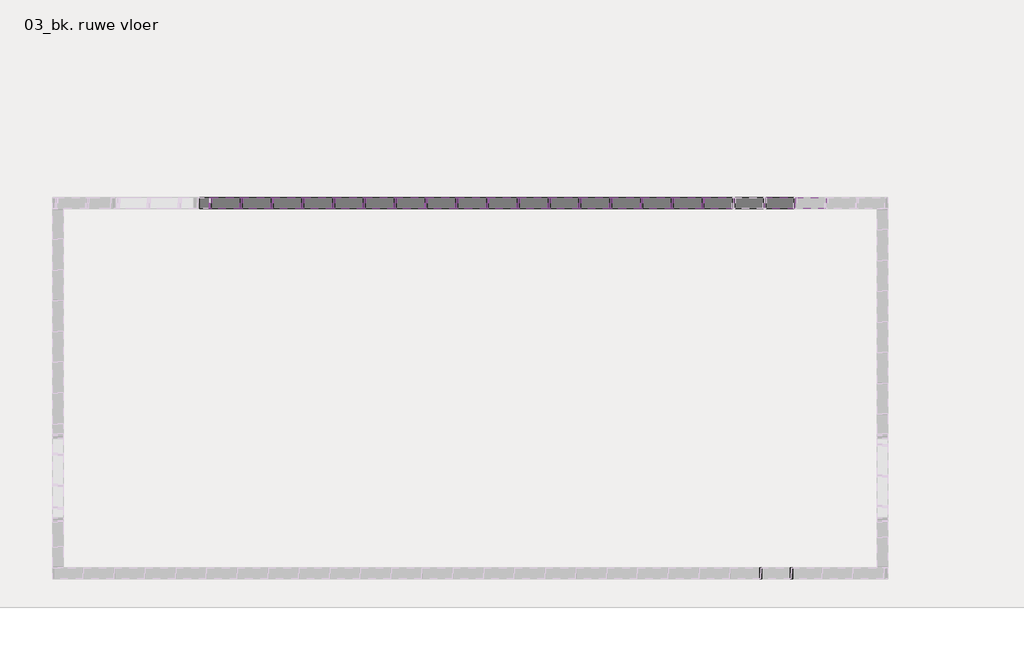
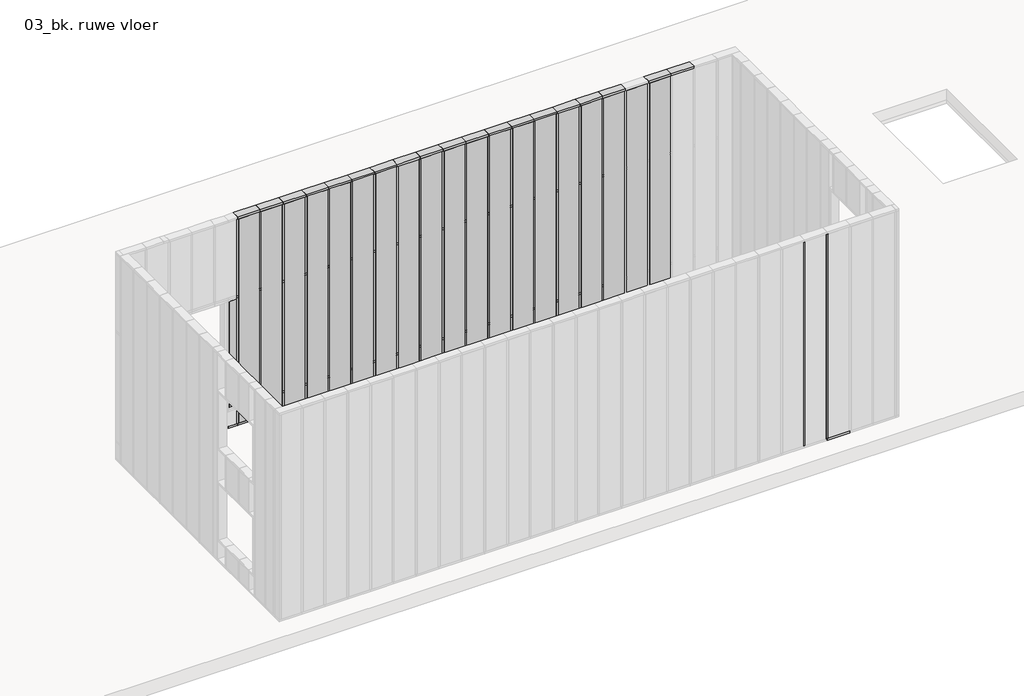
# One storey, part 3 of 9: 124 members, 20 plates.
# Revit data of these elements (continued)
# Type "Rectangular Mullion : NLRS_21_CWM_hsb-regel 38x142_gen_rsf"
#   Export Type to IFC As = "IfcWall"
#   Type IfcGUID = "07M7mRoiH1CR8m_RSKIwpF"
#   Assembly Code = "21.10"
#   built-in parameter 1007322 = 0.465879 (stored number, unit not read)
#   built-in parameter 1007321 = 0.062336 (stored number, unit not read)
#   built-in parameter 1007320 = 0.062336 (stored number, unit not read)
# Type "System Panel : NLRS_21_CWP_hsb-vulling minerale wol 142 _gen_rsf"
#   Export Type to IFC As = "IfcWall"
#   Type IfcGUID = "07M7mRoiH1CR8m_RSKIwpC"
#   Assembly Code = "21.23"
# Element 1 (IfcMember, "Rectangular Mullion : NLRS_21_CWM_hsb-regel 38x142_gen_rsf")
#   IfcGUID = "07M7mRoiH1CR8m_RSKIwQK"
#   IsExternal = yes
#   LoadBearing = yes
#   Phase Created = NLRS_nieuw
#   Materials on its faces: "NLRS_i2_hout naaldhout vuren_gen_rsf"
# Element 2 (IfcMember, "Rectangular Mullion : NLRS_21_CWM_hsb-regel 38x142_gen_rsf")
#   IfcGUID = "07M7mRoiH1CR8m_RSKIwQR"
#   IsExternal = yes
#   LoadBearing = yes
#   Phase Created = NLRS_nieuw
#   Materials on its faces: "NLRS_i2_hout naaldhout vuren_gen_rsf"
# Element 3 (IfcMember, "Rectangular Mullion : NLRS_21_CWM_hsb-regel 38x142_gen_rsf")
#   IfcGUID = "07M7mRoiH1CR8m_RSKIwQP"
#   IsExternal = yes
#   LoadBearing = yes
#   Phase Created = NLRS_nieuw
#   Materials on its faces: "NLRS_i2_hout naaldhout vuren_gen_rsf"
# Element 4 (IfcMember, "Rectangular Mullion : NLRS_21_CWM_hsb-regel 38x142_gen_rsf")
#   IfcGUID = "07M7mRoiH1CR8m_RSKIwQO"
#   IsExternal = yes
#   LoadBearing = yes
#   Phase Created = NLRS_nieuw
#   Materials on its faces: "NLRS_i2_hout naaldhout vuren_gen_rsf"
# Element 5 (IfcMember, "Rectangular Mullion : NLRS_21_CWM_hsb-regel 38x142_gen_rsf")
#   IfcGUID = "07M7mRoiH1CR8m_RSKIwQV"
#   IsExternal = yes
#   LoadBearing = yes
#   Phase Created = NLRS_nieuw
#   Materials on its faces: "NLRS_i2_hout naaldhout vuren_gen_rsf"
# Element 6 (IfcMember, "Rectangular Mullion : NLRS_21_CWM_hsb-regel 38x142_gen_rsf")
#   IfcGUID = "07M7mRoiH1CR8m_RSKIwQU"
#   IsExternal = yes
#   LoadBearing = yes
#   Phase Created = NLRS_nieuw
#   Materials on its faces: "NLRS_i2_hout naaldhout vuren_gen_rsf"
# Element 7 (IfcMember, "Rectangular Mullion : NLRS_21_CWM_hsb-regel 38x142_gen_rsf")
#   IfcGUID = "07M7mRoiH1CR8m_RSKIwQT"
#   IsExternal = yes
#   LoadBearing = yes
#   Phase Created = NLRS_nieuw
#   Materials on its faces: "NLRS_i2_hout naaldhout vuren_gen_rsf"
# Element 8 (IfcMember, "Rectangular Mullion : NLRS_21_CWM_hsb-regel 38x142_gen_rsf")
#   IfcGUID = "07M7mRoiH1CR8m_RSKIwQS"
#   IsExternal = yes
#   LoadBearing = yes
#   Phase Created = NLRS_nieuw
#   Materials on its faces: "NLRS_i2_hout naaldhout vuren_gen_rsf"
# Element 9 (IfcMember, "Rectangular Mullion : NLRS_21_CWM_hsb-regel 38x142_gen_rsf")
#   IfcGUID = "07M7mRoiH1CR8m_RSKIwPZ"
#   IsExternal = yes
#   LoadBearing = yes
#   Phase Created = NLRS_nieuw
#   Materials on its faces: "NLRS_i2_hout naaldhout vuren_gen_rsf"
# Element 10 (IfcMember, "Rectangular Mullion : NLRS_21_CWM_hsb-regel 38x142_gen_rsf")
#   IfcGUID = "07M7mRoiH1CR8m_RSKIwPY"
#   IsExternal = yes
#   LoadBearing = yes
#   Phase Created = NLRS_nieuw
#   Materials on its faces: "NLRS_i2_hout naaldhout vuren_gen_rsf"
# Element 11 (IfcMember, "Rectangular Mullion : NLRS_21_CWM_hsb-regel 38x142_gen_rsf")
#   IfcGUID = "07M7mRoiH1CR8m_RSKIwPX"
#   IsExternal = yes
#   LoadBearing = yes
#   Phase Created = NLRS_nieuw
#   Materials on its faces: "NLRS_i2_hout naaldhout vuren_gen_rsf"
# Element 12 (IfcMember, "Rectangular Mullion : NLRS_21_CWM_hsb-regel 38x142_gen_rsf")
#   IfcGUID = "07M7mRoiH1CR8m_RSKIwPW"
#   IsExternal = yes
#   LoadBearing = yes
#   Phase Created = NLRS_nieuw
#   Materials on its faces: "NLRS_i2_hout naaldhout vuren_gen_rsf"
# Element 13 (IfcMember, "Rectangular Mullion : NLRS_21_CWM_hsb-regel 38x142_gen_rsf")
#   IfcGUID = "07M7mRoiH1CR8m_RSKIwPd"
#   IsExternal = yes
#   LoadBearing = yes
#   Phase Created = NLRS_nieuw
#   Materials on its faces: "NLRS_i2_hout naaldhout vuren_gen_rsf"
# Element 14 (IfcMember, "Rectangular Mullion : NLRS_21_CWM_hsb-regel 38x142_gen_rsf")
#   IfcGUID = "07M7mRoiH1CR8m_RSKIwPc"
#   IsExternal = yes
#   LoadBearing = yes
#   Phase Created = NLRS_nieuw
#   Materials on its faces: "NLRS_i2_hout naaldhout vuren_gen_rsf"
# Element 15 (IfcMember, "Rectangular Mullion : NLRS_21_CWM_hsb-regel 38x142_gen_rsf")
#   IfcGUID = "07M7mRoiH1CR8m_RSKIwPb"
#   IsExternal = yes
#   LoadBearing = yes
#   Phase Created = NLRS_nieuw
#   Materials on its faces: "NLRS_i2_hout naaldhout vuren_gen_rsf"
# Element 16 (IfcMember, "Rectangular Mullion : NLRS_21_CWM_hsb-regel 38x142_gen_rsf")
#   IfcGUID = "07M7mRoiH1CR8m_RSKIwPa"
#   IsExternal = yes
#   LoadBearing = yes
#   Phase Created = NLRS_nieuw
#   Materials on its faces: "NLRS_i2_hout naaldhout vuren_gen_rsf"
# Element 17 (IfcMember, "Rectangular Mullion : NLRS_21_CWM_hsb-regel 38x142_gen_rsf")
#   IfcGUID = "07M7mRoiH1CR8m_RSKIwUD"
#   IsExternal = yes
#   LoadBearing = yes
#   Phase Created = NLRS_nieuw
#   Materials on its faces: "NLRS_i2_hout naaldhout vuren_gen_rsf"
# Element 18 (IfcMember, "Rectangular Mullion : NLRS_21_CWM_hsb-regel 38x142_gen_rsf")
#   IfcGUID = "07M7mRoiH1CR8m_RSKIwUC"
#   IsExternal = yes
#   LoadBearing = yes
#   Phase Created = NLRS_nieuw
#   Materials on its faces: "NLRS_i2_hout naaldhout vuren_gen_rsf"
# Element 19 (IfcMember, "Rectangular Mullion : NLRS_21_CWM_hsb-regel 38x142_gen_rsf")
#   IfcGUID = "07M7mRoiH1CR8m_RSKIwIM"
#   IsExternal = yes
#   LoadBearing = yes
#   Phase Created = NLRS_nieuw
#   Materials on its faces: "NLRS_i2_hout naaldhout vuren_gen_rsf"
# Element 20 (IfcMember, "Rectangular Mullion : NLRS_21_CWM_hsb-regel 38x142_gen_rsf")
#   IfcGUID = "07M7mRoiH1CR8m_RSKIwPj"
#   IsExternal = yes
#   LoadBearing = yes
#   Phase Created = NLRS_nieuw
#   Materials on its faces: "NLRS_i2_hout naaldhout vuren_gen_rsf"
# Element 21 (IfcMember, "Rectangular Mullion : NLRS_21_CWM_hsb-regel 38x142_gen_rsf")
#   IfcGUID = "07M7mRoiH1CR8m_RSKIwPi"
#   IsExternal = yes
#   LoadBearing = yes
#   Phase Created = NLRS_nieuw
#   Materials on its faces: "NLRS_i2_hout naaldhout vuren_gen_rsf"
# Element 22 (IfcMember, "Rectangular Mullion : NLRS_21_CWM_hsb-regel 38x142_gen_rsf")
#   IfcGUID = "07M7mRoiH1CR8m_RSKIwPp"
#   IsExternal = yes
#   LoadBearing = yes
#   Phase Created = NLRS_nieuw
#   Materials on its faces: "NLRS_i2_hout naaldhout vuren_gen_rsf"
# Element 23 (IfcMember, "Rectangular Mullion : NLRS_21_CWM_hsb-regel 38x142_gen_rsf")
#   IfcGUID = "07M7mRoiH1CR8m_RSKIwPo"
#   IsExternal = yes
#   LoadBearing = yes
#   Phase Created = NLRS_nieuw
#   Materials on its faces: "NLRS_i2_hout naaldhout vuren_gen_rsf"
# Element 24 (IfcMember, "Rectangular Mullion : NLRS_21_CWM_hsb-regel 38x142_gen_rsf")
#   IfcGUID = "07M7mRoiH1CR8m_RSKIwPn"
#   IsExternal = yes
#   LoadBearing = yes
#   Phase Created = NLRS_nieuw
#   Materials on its faces: "NLRS_i2_hout naaldhout vuren_gen_rsf"
# Element 25 (IfcMember, "Rectangular Mullion : NLRS_21_CWM_hsb-regel 38x142_gen_rsf")
#   IfcGUID = "07M7mRoiH1CR8m_RSKIwPm"
#   IsExternal = yes
#   LoadBearing = yes
#   Phase Created = NLRS_nieuw
#   Materials on its faces: "NLRS_i2_hout naaldhout vuren_gen_rsf"
# Element 26 (IfcMember, "Rectangular Mullion : NLRS_21_CWM_hsb-regel 38x142_gen_rsf")
#   IfcGUID = "07M7mRoiH1CR8m_RSKIwPt"
#   IsExternal = yes
#   LoadBearing = yes
#   Phase Created = NLRS_nieuw
#   Materials on its faces: "NLRS_i2_hout naaldhout vuren_gen_rsf"
# Element 27 (IfcMember, "Rectangular Mullion : NLRS_21_CWM_hsb-regel 38x142_gen_rsf")
#   IfcGUID = "07M7mRoiH1CR8m_RSKIwPs"
#   IsExternal = yes
#   LoadBearing = yes
#   Phase Created = NLRS_nieuw
#   Materials on its faces: "NLRS_i2_hout naaldhout vuren_gen_rsf"
# Element 28 (IfcMember, "Rectangular Mullion : NLRS_21_CWM_hsb-regel 38x142_gen_rsf")
#   IfcGUID = "07M7mRoiH1CR8m_RSKIwPr"
#   IsExternal = yes
#   LoadBearing = yes
#   Phase Created = NLRS_nieuw
#   Materials on its faces: "NLRS_i2_hout naaldhout vuren_gen_rsf"
# Element 29 (IfcMember, "Rectangular Mullion : NLRS_21_CWM_hsb-regel 38x142_gen_rsf")
#   IfcGUID = "07M7mRoiH1CR8m_RSKIwPq"
#   IsExternal = yes
#   LoadBearing = yes
#   Phase Created = NLRS_nieuw
#   Materials on its faces: "NLRS_i2_hout naaldhout vuren_gen_rsf"
# Element 30 (IfcMember, "Rectangular Mullion : NLRS_21_CWM_hsb-regel 38x142_gen_rsf")
#   IfcGUID = "07M7mRoiH1CR8m_RSKIwPx"
#   IsExternal = yes
#   LoadBearing = yes
#   Phase Created = NLRS_nieuw
#   Materials on its faces: "NLRS_i2_hout naaldhout vuren_gen_rsf"
# Element 31 (IfcMember, "Rectangular Mullion : NLRS_21_CWM_hsb-regel 38x142_gen_rsf")
#   IfcGUID = "07M7mRoiH1CR8m_RSKIwPw"
#   IsExternal = yes
#   LoadBearing = yes
#   Phase Created = NLRS_nieuw
#   Materials on its faces: "NLRS_i2_hout naaldhout vuren_gen_rsf"
# Element 32 (IfcMember, "Rectangular Mullion : NLRS_21_CWM_hsb-regel 38x142_gen_rsf")
#   IfcGUID = "07M7mRoiH1CR8m_RSKIwPv"
#   IsExternal = yes
#   LoadBearing = yes
#   Phase Created = NLRS_nieuw
#   Materials on its faces: "NLRS_i2_hout naaldhout vuren_gen_rsf"
# Element 33 (IfcMember, "Rectangular Mullion : NLRS_21_CWM_hsb-regel 38x142_gen_rsf")
#   IfcGUID = "07M7mRoiH1CR8m_RSKIwPu"
#   IsExternal = yes
#   LoadBearing = yes
#   Phase Created = NLRS_nieuw
#   Materials on its faces: "NLRS_i2_hout naaldhout vuren_gen_rsf"
# Element 34 (IfcMember, "Rectangular Mullion : NLRS_21_CWM_hsb-regel 38x142_gen_rsf")
#   IfcGUID = "07M7mRoiH1CR8m_RSKIwUJ"
#   IsExternal = yes
#   LoadBearing = yes
#   Phase Created = NLRS_nieuw
#   Materials on its faces: "NLRS_i2_hout naaldhout vuren_gen_rsf"
# Element 35 (IfcMember, "Rectangular Mullion : NLRS_21_CWM_hsb-regel 38x142_gen_rsf")
#   IfcGUID = "07M7mRoiH1CR8m_RSKIwJV"
#   IsExternal = yes
#   LoadBearing = yes
#   Phase Created = NLRS_nieuw
#   Materials on its faces: "NLRS_i2_hout naaldhout vuren_gen_rsf"
# Element 36 (IfcMember, "Rectangular Mullion : NLRS_21_CWM_hsb-regel 38x142_gen_rsf")
#   IfcGUID = "3JRv6RmLn4$9gi2tFo70EI"
#   IsExternal = yes
#   LoadBearing = yes
#   Phase Created = NLRS_nieuw
#   Materials on its faces: "NLRS_i2_hout naaldhout vuren_gen_rsf"
# Element 37 (IfcMember, "Rectangular Mullion : NLRS_21_CWM_hsb-regel 38x142_gen_rsf")
#   IfcGUID = "07M7mRoiH1CR8m_RSKIwIY"
#   IsExternal = yes
#   LoadBearing = yes
#   Phase Created = NLRS_nieuw
#   Materials on its faces: "NLRS_i2_hout naaldhout vuren_gen_rsf"
# Element 38 (IfcMember, "Rectangular Mullion : NLRS_21_CWM_hsb-regel 38x142_gen_rsf")
#   IfcGUID = "07M7mRoiH1CR8m_RSKIwIX"
#   IsExternal = yes
#   LoadBearing = yes
#   Phase Created = NLRS_nieuw
#   Materials on its faces: "NLRS_i2_hout naaldhout vuren_gen_rsf"
# Element 39 (IfcMember, "Rectangular Mullion : NLRS_21_CWM_hsb-regel 38x142_gen_rsf")
#   IfcGUID = "07M7mRoiH1CR8m_RSKIwP0"
#   IsExternal = yes
#   LoadBearing = yes
#   Phase Created = NLRS_nieuw
#   Materials on its faces: "NLRS_i2_hout naaldhout vuren_gen_rsf"
# Element 40 (IfcMember, "Rectangular Mullion : NLRS_21_CWM_hsb-regel 38x142_gen_rsf")
#   IfcGUID = "07M7mRoiH1CR8m_RSKIwP7"
#   IsExternal = yes
#   LoadBearing = yes
#   Phase Created = NLRS_nieuw
#   Materials on its faces: "NLRS_i2_hout naaldhout vuren_gen_rsf"
# Element 41 (IfcMember, "Rectangular Mullion : NLRS_21_CWM_hsb-regel 38x142_gen_rsf")
#   IfcGUID = "07M7mRoiH1CR8m_RSKIwP6"
#   IsExternal = yes
#   LoadBearing = yes
#   Phase Created = NLRS_nieuw
#   Materials on its faces: "NLRS_i2_hout naaldhout vuren_gen_rsf"
# Element 42 (IfcMember, "Rectangular Mullion : NLRS_21_CWM_hsb-regel 38x142_gen_rsf")
#   IfcGUID = "07M7mRoiH1CR8m_RSKIwP5"
#   IsExternal = yes
#   LoadBearing = yes
#   Phase Created = NLRS_nieuw
#   Materials on its faces: "NLRS_i2_hout naaldhout vuren_gen_rsf"
# Element 43 (IfcMember, "Rectangular Mullion : NLRS_21_CWM_hsb-regel 38x142_gen_rsf")
#   IfcGUID = "07M7mRoiH1CR8m_RSKIwP4"
#   IsExternal = yes
#   LoadBearing = yes
#   Phase Created = NLRS_nieuw
#   Materials on its faces: "NLRS_i2_hout naaldhout vuren_gen_rsf"
# Element 44 (IfcMember, "Rectangular Mullion : NLRS_21_CWM_hsb-regel 38x142_gen_rsf")
#   IfcGUID = "07M7mRoiH1CR8m_RSKIwPB"
#   IsExternal = yes
#   LoadBearing = yes
#   Phase Created = NLRS_nieuw
#   Materials on its faces: "NLRS_i2_hout naaldhout vuren_gen_rsf"
# Element 45 (IfcMember, "Rectangular Mullion : NLRS_21_CWM_hsb-regel 38x142_gen_rsf")
#   IfcGUID = "07M7mRoiH1CR8m_RSKIwPA"
#   IsExternal = yes
#   LoadBearing = yes
#   Phase Created = NLRS_nieuw
#   Materials on its faces: "NLRS_i2_hout naaldhout vuren_gen_rsf"
# Element 46 (IfcMember, "Rectangular Mullion : NLRS_21_CWM_hsb-regel 38x142_gen_rsf")
#   IfcGUID = "07M7mRoiH1CR8m_RSKIwP9"
#   IsExternal = yes
#   LoadBearing = yes
#   Phase Created = NLRS_nieuw
#   Materials on its faces: "NLRS_i2_hout naaldhout vuren_gen_rsf"
# Element 47 (IfcMember, "Rectangular Mullion : NLRS_21_CWM_hsb-regel 38x142_gen_rsf")
#   IfcGUID = "07M7mRoiH1CR8m_RSKIwP8"
#   IsExternal = yes
#   LoadBearing = yes
#   Phase Created = NLRS_nieuw
#   Materials on its faces: "NLRS_i2_hout naaldhout vuren_gen_rsf"
# Element 48 (IfcMember, "Rectangular Mullion : NLRS_21_CWM_hsb-regel 38x142_gen_rsf")
#   IfcGUID = "07M7mRoiH1CR8m_RSKIwPF"
#   IsExternal = yes
#   LoadBearing = yes
#   Phase Created = NLRS_nieuw
#   Materials on its faces: "NLRS_i2_hout naaldhout vuren_gen_rsf"
# Element 49 (IfcMember, "Rectangular Mullion : NLRS_21_CWM_hsb-regel 38x142_gen_rsf")
#   IfcGUID = "07M7mRoiH1CR8m_RSKIwPE"
#   IsExternal = yes
#   LoadBearing = yes
#   Phase Created = NLRS_nieuw
#   Materials on its faces: "NLRS_i2_hout naaldhout vuren_gen_rsf"
# Element 50 (IfcMember, "Rectangular Mullion : NLRS_21_CWM_hsb-regel 38x142_gen_rsf")
#   IfcGUID = "07M7mRoiH1CR8m_RSKIwPD"
#   IsExternal = yes
#   LoadBearing = yes
#   Phase Created = NLRS_nieuw
#   Materials on its faces: "NLRS_i2_hout naaldhout vuren_gen_rsf"
# Element 51 (IfcMember, "Rectangular Mullion : NLRS_21_CWM_hsb-regel 38x142_gen_rsf")
#   IfcGUID = "07M7mRoiH1CR8m_RSKIwPC"
#   IsExternal = yes
#   LoadBearing = yes
#   Phase Created = NLRS_nieuw
#   Materials on its faces: "NLRS_i2_hout naaldhout vuren_gen_rsf"
# Element 52 (IfcMember, "Rectangular Mullion : NLRS_21_CWM_hsb-regel 38x142_gen_rsf")
#   IfcGUID = "07M7mRoiH1CR8m_RSKIwPJ"
#   IsExternal = yes
#   LoadBearing = yes
#   Phase Created = NLRS_nieuw
#   Materials on its faces: "NLRS_i2_hout naaldhout vuren_gen_rsf"
# Element 53 (IfcMember, "Rectangular Mullion : NLRS_21_CWM_hsb-regel 38x142_gen_rsf")
#   IfcGUID = "07M7mRoiH1CR8m_RSKIwUI"
#   IsExternal = yes
#   LoadBearing = yes
#   Phase Created = NLRS_nieuw
#   Materials on its faces: "NLRS_i2_hout naaldhout vuren_gen_rsf"
# Element 54 (IfcMember, "Rectangular Mullion : NLRS_21_CWM_hsb-regel 38x142_gen_rsf")
#   IfcGUID = "07M7mRoiH1CR8m_RSKIwUH"
#   IsExternal = yes
#   LoadBearing = yes
#   Phase Created = NLRS_nieuw
#   Materials on its faces: "NLRS_i2_hout naaldhout vuren_gen_rsf"
# Element 55 (IfcMember, "Rectangular Mullion : NLRS_21_CWM_hsb-regel 38x142_gen_rsf")
#   IfcGUID = "07M7mRoiH1CR8m_RSKIwHY"
#   IsExternal = yes
#   LoadBearing = yes
#   Phase Created = NLRS_nieuw
#   Materials on its faces: "NLRS_i2_hout naaldhout vuren_gen_rsf"
# Element 56 (IfcMember, "Rectangular Mullion : NLRS_21_CWM_hsb-regel 38x142_gen_rsf")
#   IfcGUID = "3JRv6RmLn4$9gi2tFo70EJ"
#   IsExternal = yes
#   LoadBearing = yes
#   Phase Created = NLRS_nieuw
#   Materials on its faces: "NLRS_i2_hout naaldhout vuren_gen_rsf"
# Element 57 (IfcMember, "Rectangular Mullion : NLRS_21_CWM_hsb-regel 38x142_gen_rsf")
#   IfcGUID = "3JRv6RmLn4$9gi2tFo70WL"
#   IsExternal = yes
#   LoadBearing = yes
#   Phase Created = NLRS_nieuw
#   Materials on its faces: "NLRS_i2_hout naaldhout vuren_gen_rsf"
# Element 58 (IfcMember, "Rectangular Mullion : NLRS_21_CWM_hsb-regel 38x142_gen_rsf")
#   IfcGUID = "3JRv6RmLn4$9gi2tFo70WM"
#   IsExternal = yes
#   LoadBearing = yes
#   Phase Created = NLRS_nieuw
#   Materials on its faces: "NLRS_i2_hout naaldhout vuren_gen_rsf"
# Element 59 (IfcMember, "Rectangular Mullion : NLRS_21_CWM_hsb-regel 38x142_gen_rsf")
#   IfcGUID = "3JRv6RmLn4$9gi2tFo70WN"
#   IsExternal = yes
#   LoadBearing = yes
#   Phase Created = NLRS_nieuw
#   Materials on its faces: "NLRS_i2_hout naaldhout vuren_gen_rsf"
# Element 60 (IfcMember, "Rectangular Mullion : NLRS_21_CWM_hsb-regel 38x142_gen_rsf")
#   IfcGUID = "3JRv6RmLn4$9gi2tFo70WG"
#   IsExternal = yes
#   LoadBearing = yes
#   Phase Created = NLRS_nieuw
#   Materials on its faces: "NLRS_i2_hout naaldhout vuren_gen_rsf"
# Element 61 (IfcMember, "Rectangular Mullion : NLRS_21_CWM_hsb-regel 38x142_gen_rsf")
#   IfcGUID = "3JRv6RmLn4$9gi2tFo70WH"
#   IsExternal = yes
#   LoadBearing = yes
#   Phase Created = NLRS_nieuw
#   Materials on its faces: "NLRS_i2_hout naaldhout vuren_gen_rsf"
# Element 62 (IfcMember, "Rectangular Mullion : NLRS_21_CWM_hsb-regel 38x142_gen_rsf")
#   IfcGUID = "3JRv6RmLn4$9gi2tFo70WI"
#   IsExternal = yes
#   LoadBearing = yes
#   Phase Created = NLRS_nieuw
#   Materials on its faces: "NLRS_i2_hout naaldhout vuren_gen_rsf"
# Element 63 (IfcMember, "Rectangular Mullion : NLRS_21_CWM_hsb-regel 38x142_gen_rsf")
#   IfcGUID = "3JRv6RmLn4$9gi2tFo70WJ"
#   IsExternal = yes
#   LoadBearing = yes
#   Phase Created = NLRS_nieuw
#   Materials on its faces: "NLRS_i2_hout naaldhout vuren_gen_rsf"
# Element 64 (IfcMember, "Rectangular Mullion : NLRS_21_CWM_hsb-regel 38x142_gen_rsf")
#   IfcGUID = "3JRv6RmLn4$9gi2tFo70WS"
#   IsExternal = yes
#   LoadBearing = yes
#   Phase Created = NLRS_nieuw
#   Materials on its faces: "NLRS_i2_hout naaldhout vuren_gen_rsf"
# Element 65 (IfcMember, "Rectangular Mullion : NLRS_21_CWM_hsb-regel 38x142_gen_rsf")
#   IfcGUID = "3JRv6RmLn4$9gi2tFo70WT"
#   IsExternal = yes
#   LoadBearing = yes
#   Phase Created = NLRS_nieuw
#   Materials on its faces: "NLRS_i2_hout naaldhout vuren_gen_rsf"
# Element 66 (IfcMember, "Rectangular Mullion : NLRS_21_CWM_hsb-regel 38x142_gen_rsf")
#   IfcGUID = "3JRv6RmLn4$9gi2tFo70WU"
#   IsExternal = yes
#   LoadBearing = yes
#   Phase Created = NLRS_nieuw
#   Materials on its faces: "NLRS_i2_hout naaldhout vuren_gen_rsf"
# Element 67 (IfcMember, "Rectangular Mullion : NLRS_21_CWM_hsb-regel 38x142_gen_rsf")
#   IfcGUID = "3JRv6RmLn4$9gi2tFo70WV"
#   IsExternal = yes
#   LoadBearing = yes
#   Phase Created = NLRS_nieuw
#   Materials on its faces: "NLRS_i2_hout naaldhout vuren_gen_rsf"
# Element 68 (IfcMember, "Rectangular Mullion : NLRS_21_CWM_hsb-regel 38x142_gen_rsf")
#   IfcGUID = "3JRv6RmLn4$9gi2tFo70WO"
#   IsExternal = yes
#   LoadBearing = yes
#   Phase Created = NLRS_nieuw
#   Materials on its faces: "NLRS_i2_hout naaldhout vuren_gen_rsf"
# Element 69 (IfcMember, "Rectangular Mullion : NLRS_21_CWM_hsb-regel 38x142_gen_rsf")
#   IfcGUID = "3JRv6RmLn4$9gi2tFo70WP"
#   IsExternal = yes
#   LoadBearing = yes
#   Phase Created = NLRS_nieuw
#   Materials on its faces: "NLRS_i2_hout naaldhout vuren_gen_rsf"
# Element 70 (IfcMember, "Rectangular Mullion : NLRS_21_CWM_hsb-regel 38x142_gen_rsf")
#   IfcGUID = "3JRv6RmLn4$9gi2tFo70WQ"
#   IsExternal = yes
#   LoadBearing = yes
#   Phase Created = NLRS_nieuw
#   Materials on its faces: "NLRS_i2_hout naaldhout vuren_gen_rsf"
# Element 71 (IfcMember, "Rectangular Mullion : NLRS_21_CWM_hsb-regel 38x142_gen_rsf")
#   IfcGUID = "3JRv6RmLn4$9gi2tFo70WR"
#   IsExternal = yes
#   LoadBearing = yes
#   Phase Created = NLRS_nieuw
#   Materials on its faces: "NLRS_i2_hout naaldhout vuren_gen_rsf"
# Element 72 (IfcMember, "Rectangular Mullion : NLRS_21_CWM_hsb-regel 38x142_gen_rsf")
#   IfcGUID = "3JRv6RmLn4$9gi2tFo70Xa"
#   IsExternal = yes
#   LoadBearing = yes
#   Phase Created = NLRS_nieuw
#   Materials on its faces: "NLRS_i2_hout naaldhout vuren_gen_rsf"
# Element 73 (IfcMember, "Rectangular Mullion : NLRS_21_CWM_hsb-regel 38x142_gen_rsf")
#   IfcGUID = "3JRv6RmLn4$9gi2tFo70Xb"
#   IsExternal = yes
#   LoadBearing = yes
#   Phase Created = NLRS_nieuw
#   Materials on its faces: "NLRS_i2_hout naaldhout vuren_gen_rsf"
# Element 74 (IfcMember, "Rectangular Mullion : NLRS_21_CWM_hsb-regel 38x142_gen_rsf")
#   IfcGUID = "3JRv6RmLn4$9gi2tFo70wj"
#   IsExternal = yes
#   LoadBearing = yes
#   Phase Created = NLRS_nieuw
#   Materials on its faces: "NLRS_i2_hout naaldhout vuren_gen_rsf"
# Element 75 (IfcMember, "Rectangular Mullion : NLRS_21_CWM_hsb-regel 38x142_gen_rsf")
#   IfcGUID = "3JRv6RmLn4$9gi2tFo70wk"
#   IsExternal = yes
#   LoadBearing = yes
#   Phase Created = NLRS_nieuw
#   Materials on its faces: "NLRS_i2_hout naaldhout vuren_gen_rsf"
# Element 76 (IfcMember, "Rectangular Mullion : NLRS_21_CWM_hsb-regel 38x142_gen_rsf")
#   IfcGUID = "3JRv6RmLn4$9gi2tFo70wl"
#   IsExternal = yes
#   LoadBearing = yes
#   Phase Created = NLRS_nieuw
#   Materials on its faces: "NLRS_i2_hout naaldhout vuren_gen_rsf"
# Element 77 (IfcMember, "Rectangular Mullion : NLRS_21_CWM_hsb-regel 38x142_gen_rsf")
#   IfcGUID = "3JRv6RmLn4$9gi2tFo70we"
#   IsExternal = yes
#   LoadBearing = yes
#   Phase Created = NLRS_nieuw
#   Materials on its faces: "NLRS_i2_hout naaldhout vuren_gen_rsf"
# Element 78 (IfcMember, "Rectangular Mullion : NLRS_21_CWM_hsb-regel 38x142_gen_rsf")
#   IfcGUID = "3JRv6RmLn4$9gi2tFo70wf"
#   IsExternal = yes
#   LoadBearing = yes
#   Phase Created = NLRS_nieuw
#   Materials on its faces: "NLRS_i2_hout naaldhout vuren_gen_rsf"
# Element 79 (IfcMember, "Rectangular Mullion : NLRS_21_CWM_hsb-regel 38x142_gen_rsf")
#   IfcGUID = "3JRv6RmLn4$9gi2tFo70wg"
#   IsExternal = yes
#   LoadBearing = yes
#   Phase Created = NLRS_nieuw
#   Materials on its faces: "NLRS_i2_hout naaldhout vuren_gen_rsf"
# Element 80 (IfcMember, "Rectangular Mullion : NLRS_21_CWM_hsb-regel 38x142_gen_rsf")
#   IfcGUID = "3JRv6RmLn4$9gi2tFo70wh"
#   IsExternal = yes
#   LoadBearing = yes
#   Phase Created = NLRS_nieuw
#   Materials on its faces: "NLRS_i2_hout naaldhout vuren_gen_rsf"
# Element 81 (IfcMember, "Rectangular Mullion : NLRS_21_CWM_hsb-regel 38x142_gen_rsf")
#   IfcGUID = "3JRv6RmLn4$9gi2tFo70wq"
#   IsExternal = yes
#   LoadBearing = yes
#   Phase Created = NLRS_nieuw
#   Materials on its faces: "NLRS_i2_hout naaldhout vuren_gen_rsf"
# Element 82 (IfcMember, "Rectangular Mullion : NLRS_21_CWM_hsb-regel 38x142_gen_rsf")
#   IfcGUID = "3JRv6RmLn4$9gi2tFo70wr"
#   IsExternal = yes
#   LoadBearing = yes
#   Phase Created = NLRS_nieuw
#   Materials on its faces: "NLRS_i2_hout naaldhout vuren_gen_rsf"
# Element 83 (IfcMember, "Rectangular Mullion : NLRS_21_CWM_hsb-regel 38x142_gen_rsf")
#   IfcGUID = "3JRv6RmLn4$9gi2tFo70ws"
#   IsExternal = yes
#   LoadBearing = yes
#   Phase Created = NLRS_nieuw
#   Materials on its faces: "NLRS_i2_hout naaldhout vuren_gen_rsf"
# Element 84 (IfcMember, "Rectangular Mullion : NLRS_21_CWM_hsb-regel 38x142_gen_rsf")
#   IfcGUID = "3JRv6RmLn4$9gi2tFo70wt"
#   IsExternal = yes
#   LoadBearing = yes
#   Phase Created = NLRS_nieuw
#   Materials on its faces: "NLRS_i2_hout naaldhout vuren_gen_rsf"
# Element 85 (IfcMember, "Rectangular Mullion : NLRS_21_CWM_hsb-regel 38x142_gen_rsf")
#   IfcGUID = "3JRv6RmLn4$9gi2tFo70wm"
#   IsExternal = yes
#   LoadBearing = yes
#   Phase Created = NLRS_nieuw
#   Materials on its faces: "NLRS_i2_hout naaldhout vuren_gen_rsf"
# Element 86 (IfcMember, "Rectangular Mullion : NLRS_21_CWM_hsb-regel 38x142_gen_rsf")
#   IfcGUID = "3JRv6RmLn4$9gi2tFo70wn"
#   IsExternal = yes
#   LoadBearing = yes
#   Phase Created = NLRS_nieuw
#   Materials on its faces: "NLRS_i2_hout naaldhout vuren_gen_rsf"
# Element 87 (IfcMember, "Rectangular Mullion : NLRS_21_CWM_hsb-regel 38x142_gen_rsf")
#   IfcGUID = "3JRv6RmLn4$9gi2tFo70wo"
#   IsExternal = yes
#   LoadBearing = yes
#   Phase Created = NLRS_nieuw
#   Materials on its faces: "NLRS_i2_hout naaldhout vuren_gen_rsf"
# Element 88 (IfcMember, "Rectangular Mullion : NLRS_21_CWM_hsb-regel 38x142_gen_rsf")
#   IfcGUID = "3JRv6RmLn4$9gi2tFo70wp"
#   IsExternal = yes
#   LoadBearing = yes
#   Phase Created = NLRS_nieuw
#   Materials on its faces: "NLRS_i2_hout naaldhout vuren_gen_rsf"
# Element 89 (IfcMember, "Rectangular Mullion : NLRS_21_CWM_hsb-regel 38x142_gen_rsf")
#   IfcGUID = "3JRv6RmLn4$9gi2tFo70wy"
#   IsExternal = yes
#   LoadBearing = yes
#   Phase Created = NLRS_nieuw
#   Materials on its faces: "NLRS_i2_hout naaldhout vuren_gen_rsf"
# Element 90 (IfcMember, "Rectangular Mullion : NLRS_21_CWM_hsb-regel 38x142_gen_rsf")
#   IfcGUID = "3JRv6RmLn4$9gi2tFo70hi"
#   IsExternal = yes
#   LoadBearing = yes
#   Phase Created = NLRS_nieuw
#   Materials on its faces: "NLRS_i2_hout naaldhout vuren_gen_rsf"
# Element 91 (IfcMember, "Rectangular Mullion : NLRS_21_CWM_hsb-regel 38x142_gen_rsf")
#   IfcGUID = "3JRv6RmLn4$9gi2tFo70hj"
#   IsExternal = yes
#   LoadBearing = yes
#   Phase Created = NLRS_nieuw
#   Materials on its faces: "NLRS_i2_hout naaldhout vuren_gen_rsf"
# Element 92 (IfcMember, "Rectangular Mullion : NLRS_21_CWM_hsb-regel 38x142_gen_rsf")
#   IfcGUID = "3JRv6RmLn4$9gi2tFo70hk"
#   IsExternal = yes
#   LoadBearing = yes
#   Phase Created = NLRS_nieuw
#   Materials on its faces: "NLRS_i2_hout naaldhout vuren_gen_rsf"
# Element 93 (IfcMember, "Rectangular Mullion : NLRS_21_CWM_hsb-regel 38x142_gen_rsf")
#   IfcGUID = "3JRv6RmLn4$9gi2tFo70hl"
#   IsExternal = yes
#   LoadBearing = yes
#   Phase Created = NLRS_nieuw
#   Materials on its faces: "NLRS_i2_hout naaldhout vuren_gen_rsf"
# Element 94 (IfcMember, "Rectangular Mullion : NLRS_21_CWM_hsb-regel 38x142_gen_rsf")
#   IfcGUID = "3JRv6RmLn4$9gi2tFo70he"
#   IsExternal = yes
#   LoadBearing = yes
#   Phase Created = NLRS_nieuw
#   Materials on its faces: "NLRS_i2_hout naaldhout vuren_gen_rsf"
# Element 95 (IfcMember, "Rectangular Mullion : NLRS_21_CWM_hsb-regel 38x142_gen_rsf")
#   IfcGUID = "3JRv6RmLn4$9gi2tFo70hf"
#   IsExternal = yes
#   LoadBearing = yes
#   Phase Created = NLRS_nieuw
#   Materials on its faces: "NLRS_i2_hout naaldhout vuren_gen_rsf"
# Element 96 (IfcMember, "Rectangular Mullion : NLRS_21_CWM_hsb-regel 38x142_gen_rsf")
#   IfcGUID = "3JRv6RmLn4$9gi2tFo70hg"
#   IsExternal = yes
#   LoadBearing = yes
#   Phase Created = NLRS_nieuw
#   Materials on its faces: "NLRS_i2_hout naaldhout vuren_gen_rsf"
# Element 97 (IfcMember, "Rectangular Mullion : NLRS_21_CWM_hsb-regel 38x142_gen_rsf")
#   IfcGUID = "3JRv6RmLn4$9gi2tFo70hh"
#   IsExternal = yes
#   LoadBearing = yes
#   Phase Created = NLRS_nieuw
#   Materials on its faces: "NLRS_i2_hout naaldhout vuren_gen_rsf"
# Element 98 (IfcMember, "Rectangular Mullion : NLRS_21_CWM_hsb-regel 38x142_gen_rsf")
#   IfcGUID = "3JRv6RmLn4$9gi2tFo70hq"
#   IsExternal = yes
#   LoadBearing = yes
#   Phase Created = NLRS_nieuw
#   Materials on its faces: "NLRS_i2_hout naaldhout vuren_gen_rsf"
# Element 99 (IfcMember, "Rectangular Mullion : NLRS_21_CWM_hsb-regel 38x142_gen_rsf")
#   IfcGUID = "3JRv6RmLn4$9gi2tFo70hr"
#   IsExternal = yes
#   LoadBearing = yes
#   Phase Created = NLRS_nieuw
#   Materials on its faces: "NLRS_i2_hout naaldhout vuren_gen_rsf"
# Element 100 (IfcMember, "Rectangular Mullion : NLRS_21_CWM_hsb-regel 38x142_gen_rsf")
#   IfcGUID = "3JRv6RmLn4$9gi2tFo70hs"
#   IsExternal = yes
#   LoadBearing = yes
#   Phase Created = NLRS_nieuw
#   Materials on its faces: "NLRS_i2_hout naaldhout vuren_gen_rsf"
# Element 101 (IfcMember, "Rectangular Mullion : NLRS_21_CWM_hsb-regel 38x142_gen_rsf")
#   IfcGUID = "3JRv6RmLn4$9gi2tFo70ht"
#   IsExternal = yes
#   LoadBearing = yes
#   Phase Created = NLRS_nieuw
#   Materials on its faces: "NLRS_i2_hout naaldhout vuren_gen_rsf"
# Element 102 (IfcMember, "Rectangular Mullion : NLRS_21_CWM_hsb-regel 38x142_gen_rsf")
#   IfcGUID = "3JRv6RmLn4$9gi2tFo70hm"
#   IsExternal = yes
#   LoadBearing = yes
#   Phase Created = NLRS_nieuw
#   Materials on its faces: "NLRS_i2_hout naaldhout vuren_gen_rsf"
# Element 103 (IfcMember, "Rectangular Mullion : NLRS_21_CWM_hsb-regel 38x142_gen_rsf")
#   IfcGUID = "3JRv6RmLn4$9gi2tFo70hn"
#   IsExternal = yes
#   LoadBearing = yes
#   Phase Created = NLRS_nieuw
#   Materials on its faces: "NLRS_i2_hout naaldhout vuren_gen_rsf"
# Element 104 (IfcMember, "Rectangular Mullion : NLRS_21_CWM_hsb-regel 38x142_gen_rsf")
#   IfcGUID = "3JRv6RmLn4$9gi2tFo70ho"
#   IsExternal = yes
#   LoadBearing = yes
#   Phase Created = NLRS_nieuw
#   Materials on its faces: "NLRS_i2_hout naaldhout vuren_gen_rsf"
# Element 105 (IfcMember, "Rectangular Mullion : NLRS_21_CWM_hsb-regel 38x142_gen_rsf")
#   IfcGUID = "3JRv6RmLn4$9gi2tFo70hp"
#   IsExternal = yes
#   LoadBearing = yes
#   Phase Created = NLRS_nieuw
#   Materials on its faces: "NLRS_i2_hout naaldhout vuren_gen_rsf"
# Element 106 (IfcMember, "Rectangular Mullion : NLRS_21_CWM_hsb-regel 38x142_gen_rsf")
#   IfcGUID = "3JRv6RmLn4$9gi2tFo70wz"
#   IsExternal = yes
#   LoadBearing = yes
#   Phase Created = NLRS_nieuw
#   Materials on its faces: "NLRS_i2_hout naaldhout vuren_gen_rsf"
# Element 107 (IfcMember, "Rectangular Mullion : NLRS_21_CWM_hsb-regel 38x142_gen_rsf")
#   IfcGUID = "3JRv6RmLn4$9gi2tFo70hy"
#   IsExternal = yes
#   LoadBearing = yes
#   Phase Created = NLRS_nieuw
#   Materials on its faces: "NLRS_i2_hout naaldhout vuren_gen_rsf"
# Element 108 (IfcMember, "Rectangular Mullion : NLRS_21_CWM_hsb-regel 38x142_gen_rsf")
#   IfcGUID = "3JRv6RmLn4$9gi2tFo70kv"
#   IsExternal = yes
#   LoadBearing = yes
#   Phase Created = NLRS_nieuw
#   Materials on its faces: "NLRS_i2_hout naaldhout vuren_gen_rsf"
# Element 109 (IfcMember, "Rectangular Mullion : NLRS_21_CWM_hsb-regel 38x142_gen_rsf")
#   IfcGUID = "3JRv6RmLn4$9gi2tFo70kw"
#   IsExternal = yes
#   LoadBearing = yes
#   Phase Created = NLRS_nieuw
#   Materials on its faces: "NLRS_i2_hout naaldhout vuren_gen_rsf"
# Element 110 (IfcMember, "Rectangular Mullion : NLRS_21_CWM_hsb-regel 38x142_gen_rsf")
#   IfcGUID = "3JRv6RmLn4$9gi2tFo70kx"
#   IsExternal = yes
#   LoadBearing = yes
#   Phase Created = NLRS_nieuw
#   Materials on its faces: "NLRS_i2_hout naaldhout vuren_gen_rsf"
# Element 111 (IfcMember, "Rectangular Mullion : NLRS_21_CWM_hsb-regel 38x142_gen_rsf")
#   IfcGUID = "3JRv6RmLn4$9gi2tFo70k4"
#   IsExternal = yes
#   LoadBearing = yes
#   Phase Created = NLRS_nieuw
#   Materials on its faces: "NLRS_i2_hout naaldhout vuren_gen_rsf"
# Element 112 (IfcMember, "Rectangular Mullion : NLRS_21_CWM_hsb-regel 38x142_gen_rsf")
#   IfcGUID = "3JRv6RmLn4$9gi2tFo70k5"
#   IsExternal = yes
#   LoadBearing = yes
#   Phase Created = NLRS_nieuw
#   Materials on its faces: "NLRS_i2_hout naaldhout vuren_gen_rsf"
# Element 113 (IfcMember, "Rectangular Mullion : NLRS_21_CWM_hsb-regel 38x142_gen_rsf")
#   IfcGUID = "3JRv6RmLn4$9gi2tFo70k6"
#   IsExternal = yes
#   LoadBearing = yes
#   Phase Created = NLRS_nieuw
#   Materials on its faces: "NLRS_i2_hout naaldhout vuren_gen_rsf"
# Element 114 (IfcMember, "Rectangular Mullion : NLRS_21_CWM_hsb-regel 38x142_gen_rsf")
#   IfcGUID = "3JRv6RmLn4$9gi2tFo70k7"
#   IsExternal = yes
#   LoadBearing = yes
#   Phase Created = NLRS_nieuw
#   Materials on its faces: "NLRS_i2_hout naaldhout vuren_gen_rsf"
# Element 115 (IfcMember, "Rectangular Mullion : NLRS_21_CWM_hsb-regel 38x142_gen_rsf")
#   IfcGUID = "3JRv6RmLn4$9gi2tFo70k0"
#   IsExternal = yes
#   LoadBearing = yes
#   Phase Created = NLRS_nieuw
#   Materials on its faces: "NLRS_i2_hout naaldhout vuren_gen_rsf"
# Element 116 (IfcMember, "Rectangular Mullion : NLRS_21_CWM_hsb-regel 38x142_gen_rsf")
#   IfcGUID = "3JRv6RmLn4$9gi2tFo70k1"
#   IsExternal = yes
#   LoadBearing = yes
#   Phase Created = NLRS_nieuw
#   Materials on its faces: "NLRS_i2_hout naaldhout vuren_gen_rsf"
# Element 117 (IfcMember, "Rectangular Mullion : NLRS_21_CWM_hsb-regel 38x142_gen_rsf")
#   IfcGUID = "3JRv6RmLn4$9gi2tFo70k2"
#   IsExternal = yes
#   LoadBearing = yes
#   Phase Created = NLRS_nieuw
#   Materials on its faces: "NLRS_i2_hout naaldhout vuren_gen_rsf"
# Element 118 (IfcMember, "Rectangular Mullion : NLRS_21_CWM_hsb-regel 38x142_gen_rsf")
#   IfcGUID = "3JRv6RmLn4$9gi2tFo70k3"
#   IsExternal = yes
#   LoadBearing = yes
#   Phase Created = NLRS_nieuw
#   Materials on its faces: "NLRS_i2_hout naaldhout vuren_gen_rsf"
# Element 119 (IfcMember, "Rectangular Mullion : NLRS_21_CWM_hsb-regel 38x142_gen_rsf")
#   IfcGUID = "3JRv6RmLn4$9gi2tFo70kC"
#   IsExternal = yes
#   LoadBearing = yes
#   Phase Created = NLRS_nieuw
#   Materials on its faces: "NLRS_i2_hout naaldhout vuren_gen_rsf"
# Element 120 (IfcMember, "Rectangular Mullion : NLRS_21_CWM_hsb-regel 38x142_gen_rsf")
#   IfcGUID = "3JRv6RmLn4$9gi2tFo70kD"
#   IsExternal = yes
#   LoadBearing = yes
#   Phase Created = NLRS_nieuw
#   Materials on its faces: "NLRS_i2_hout naaldhout vuren_gen_rsf"
# Element 121 (IfcMember, "Rectangular Mullion : NLRS_21_CWM_hsb-regel 38x142_gen_rsf")
#   IfcGUID = "3JRv6RmLn4$9gi2tFo70kE"
#   IsExternal = yes
#   LoadBearing = yes
#   Phase Created = NLRS_nieuw
#   Materials on its faces: "NLRS_i2_hout naaldhout vuren_gen_rsf"
# Element 122 (IfcMember, "Rectangular Mullion : NLRS_21_CWM_hsb-regel 38x142_gen_rsf")
#   IfcGUID = "3JRv6RmLn4$9gi2tFo70kF"
#   IsExternal = yes
#   LoadBearing = yes
#   Phase Created = NLRS_nieuw
#   Materials on its faces: "NLRS_i2_hout naaldhout vuren_gen_rsf"
# Element 123 (IfcMember, "Rectangular Mullion : NLRS_21_CWM_hsb-regel 38x142_gen_rsf")
#   IfcGUID = "3JRv6RmLn4$9gi2tFo70k8"
#   IsExternal = yes
#   LoadBearing = yes
#   Phase Created = NLRS_nieuw
#   Materials on its faces: "NLRS_i2_hout naaldhout vuren_gen_rsf"
# Element 124 (IfcMember, "Rectangular Mullion : NLRS_21_CWM_hsb-regel 38x142_gen_rsf")
#   IfcGUID = "3JRv6RmLn4$9gi2tFo70k9"
#   IsExternal = yes
#   LoadBearing = yes
#   Phase Created = NLRS_nieuw
#   Materials on its faces: "NLRS_i2_hout naaldhout vuren_gen_rsf"
# Element 125 (IfcPlate, "System Panel : NLRS_21_CWP_hsb-vulling minerale wol 142 _gen_rsf")
#   IfcGUID = "07M7mRoiH1CR8m_RSKIwQt"
#   IsExternal = yes
#   LoadBearing = yes
#   Phase Created = NLRS_nieuw
#   Materials on its faces: "NLRS_m1_isolatie minerale wol_gen_rsf"
# Element 126 (IfcPlate, "System Panel : NLRS_21_CWP_hsb-vulling minerale wol 142 _gen_rsf")
#   IfcGUID = "07M7mRoiH1CR8m_RSKIwQr"
#   IsExternal = yes
#   LoadBearing = yes
#   Phase Created = NLRS_nieuw
#   Materials on its faces: "NLRS_m1_isolatie minerale wol_gen_rsf"
# Element 127 (IfcPlate, "System Panel : NLRS_21_CWP_hsb-vulling minerale wol 142 _gen_rsf")
#   IfcGUID = "07M7mRoiH1CR8m_RSKIwQx"
#   IsExternal = yes
#   LoadBearing = yes
#   Phase Created = NLRS_nieuw
#   Materials on its faces: "NLRS_m1_isolatie minerale wol_gen_rsf"
# Element 128 (IfcPlate, "System Panel : NLRS_21_CWP_hsb-vulling minerale wol 142 _gen_rsf")
#   IfcGUID = "07M7mRoiH1CR8m_RSKIwQv"
#   IsExternal = yes
#   LoadBearing = yes
#   Phase Created = NLRS_nieuw
#   Materials on its faces: "NLRS_m1_isolatie minerale wol_gen_rsf"
# Element 129 (IfcPlate, "System Panel : NLRS_21_CWP_hsb-vulling minerale wol 142 _gen_rsf")
#   IfcGUID = "07M7mRoiH1CR8m_RSKIwQ$"
#   IsExternal = yes
#   LoadBearing = yes
#   Phase Created = NLRS_nieuw
#   Materials on its faces: "NLRS_m1_isolatie minerale wol_gen_rsf"
# Element 130 (IfcPlate, "System Panel : NLRS_21_CWP_hsb-vulling minerale wol 142 _gen_rsf")
#   IfcGUID = "07M7mRoiH1CR8m_RSKIwQz"
#   IsExternal = yes
#   LoadBearing = yes
#   Phase Created = NLRS_nieuw
#   Materials on its faces: "NLRS_m1_isolatie minerale wol_gen_rsf"
# Element 131 (IfcPlate, "System Panel : NLRS_21_CWP_hsb-vulling minerale wol 142 _gen_rsf")
#   IfcGUID = "07M7mRoiH1CR8m_RSKIwQ3"
#   IsExternal = yes
#   LoadBearing = yes
#   Phase Created = NLRS_nieuw
#   Materials on its faces: "NLRS_m1_isolatie minerale wol_gen_rsf"
# Element 132 (IfcPlate, "System Panel : NLRS_21_CWP_hsb-vulling minerale wol 142 _gen_rsf")
#   IfcGUID = "07M7mRoiH1CR8m_RSKIwQ1"
#   IsExternal = yes
#   LoadBearing = yes
#   Phase Created = NLRS_nieuw
#   Materials on its faces: "NLRS_m1_isolatie minerale wol_gen_rsf"
# Element 133 (IfcPlate, "System Panel : NLRS_21_CWP_hsb-vulling minerale wol 142 _gen_rsf")
#   IfcGUID = "07M7mRoiH1CR8m_RSKIwQ7"
#   IsExternal = yes
#   LoadBearing = yes
#   Phase Created = NLRS_nieuw
#   Materials on its faces: "NLRS_m1_isolatie minerale wol_gen_rsf"
# Element 134 (IfcPlate, "System Panel : NLRS_21_CWP_hsb-vulling minerale wol 142 _gen_rsf")
#   IfcGUID = "07M7mRoiH1CR8m_RSKIwQ5"
#   IsExternal = yes
#   LoadBearing = yes
#   Phase Created = NLRS_nieuw
#   Materials on its faces: "NLRS_m1_isolatie minerale wol_gen_rsf"
# Element 135 (IfcPlate, "System Panel : NLRS_21_CWP_hsb-vulling minerale wol 142 _gen_rsf")
#   IfcGUID = "07M7mRoiH1CR8m_RSKIwQB"
#   IsExternal = yes
#   LoadBearing = yes
#   Phase Created = NLRS_nieuw
#   Materials on its faces: "NLRS_m1_isolatie minerale wol_gen_rsf"
# Element 136 (IfcPlate, "System Panel : NLRS_21_CWP_hsb-vulling minerale wol 142 _gen_rsf")
#   IfcGUID = "07M7mRoiH1CR8m_RSKIwQ9"
#   IsExternal = yes
#   LoadBearing = yes
#   Phase Created = NLRS_nieuw
#   Materials on its faces: "NLRS_m1_isolatie minerale wol_gen_rsf"
# Element 137 (IfcPlate, "System Panel : NLRS_21_CWP_hsb-vulling minerale wol 142 _gen_rsf")
#   IfcGUID = "07M7mRoiH1CR8m_RSKIwQF"
#   IsExternal = yes
#   LoadBearing = yes
#   Phase Created = NLRS_nieuw
#   Materials on its faces: "NLRS_m1_isolatie minerale wol_gen_rsf"
# Element 138 (IfcPlate, "System Panel : NLRS_21_CWP_hsb-vulling minerale wol 142 _gen_rsf")
#   IfcGUID = "07M7mRoiH1CR8m_RSKIwQD"
#   IsExternal = yes
#   LoadBearing = yes
#   Phase Created = NLRS_nieuw
#   Materials on its faces: "NLRS_m1_isolatie minerale wol_gen_rsf"
# Element 139 (IfcPlate, "System Panel : NLRS_21_CWP_hsb-vulling minerale wol 142 _gen_rsf")
#   IfcGUID = "07M7mRoiH1CR8m_RSKIwQJ"
#   IsExternal = yes
#   LoadBearing = yes
#   Phase Created = NLRS_nieuw
#   Materials on its faces: "NLRS_m1_isolatie minerale wol_gen_rsf"
# Element 140 (IfcPlate, "System Panel : NLRS_21_CWP_hsb-vulling minerale wol 142 _gen_rsf")
#   IfcGUID = "07M7mRoiH1CR8m_RSKIwQH"
#   IsExternal = yes
#   LoadBearing = yes
#   Phase Created = NLRS_nieuw
#   Materials on its faces: "NLRS_m1_isolatie minerale wol_gen_rsf"
# Element 141 (IfcPlate, "System Panel : NLRS_21_CWP_hsb-vulling minerale wol 142 _gen_rsf")
#   IfcGUID = "07M7mRoiH1CR8m_RSKIwQN"
#   IsExternal = yes
#   LoadBearing = yes
#   Phase Created = NLRS_nieuw
#   Materials on its faces: "NLRS_m1_isolatie minerale wol_gen_rsf"
# Element 142 (IfcPlate, "System Panel : NLRS_21_CWP_hsb-vulling minerale wol 142 _gen_rsf")
#   IfcGUID = "07M7mRoiH1CR8m_RSKIwU8"
#   IsExternal = yes
#   LoadBearing = yes
#   Phase Created = NLRS_nieuw
#   Materials on its faces: "NLRS_m1_isolatie minerale wol_gen_rsf"
# Element 143 (IfcPlate, "System Panel : NLRS_21_CWP_hsb-vulling minerale wol 142 _gen_rsf")
#   IfcGUID = "07M7mRoiH1CR8m_RSKIwUE"
#   IsExternal = yes
#   LoadBearing = yes
#   Phase Created = NLRS_nieuw
#   Materials on its faces: "NLRS_m1_isolatie minerale wol_gen_rsf"
# Element 144 (IfcPlate, "System Panel : NLRS_21_CWP_hsb-vulling minerale wol 142 _gen_rsf")
#   IfcGUID = "3JRv6RmLn4$9gi2tFo70j6"
#   IsExternal = yes
#   LoadBearing = yes
#   Phase Created = NLRS_nieuw
#   Materials on its faces: "NLRS_m1_isolatie minerale wol_gen_rsf"
# Materials
#   "NLRS_i2_hout naaldhout vuren_gen_rsf": class "I - Hout", colour RGB 234 199 147, transparency 0, Keynote = "i2", Manufacturer = "Revit Standards Foundation", URL = "www.revitstandards.org", Description = "hout vuren", Cost = 0
#   "NLRS_m1_isolatie minerale wol_gen_rsf": class "M - Anorganische materialen", colour RGB 200 200 140, transparency 0, Keynote = "m1", Manufacturer = "Revit Standards Foundation", URL = "www.revitstandards.org", Description = "isolatie minerale wol", Cost = 0
